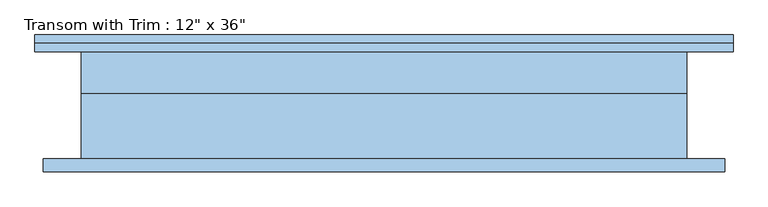
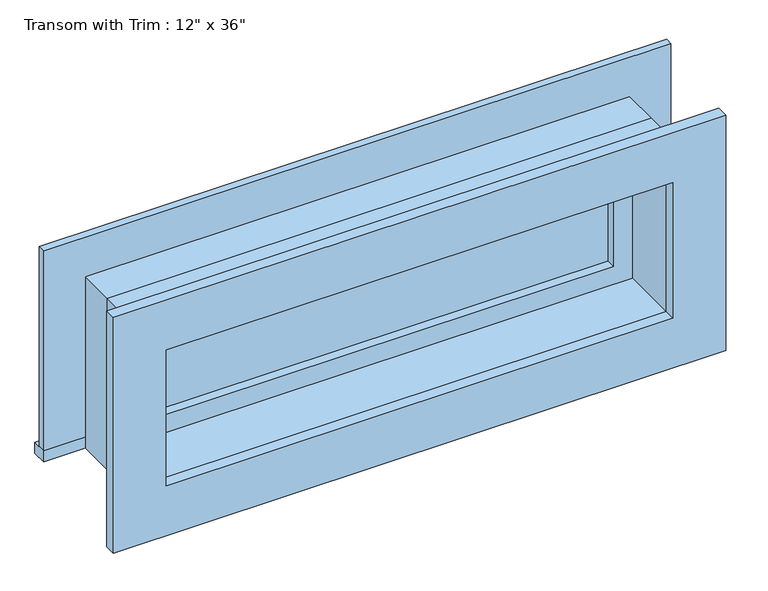
"""IFC4 building model written with IfcOpenShell, lengths in millimetres: window geometry."""

from ifc_helpers import new_model, si_unit, frame, origin, place, context, project, spatial, polyline, outline, extrude, source, transform, mapped, element, save


def window_4a3b5ce9(model_context):
    return source(origin(), model_context, "Body", "SweptSolid", [
        extrude(outline(polyline([(-565.15, 106.3625), (488.95, 106.3625), (488.95, 80.9625), (-565.15, 80.9625), (-565.15, 106.3625)])), frame((0.0, 0.0, 2159.0), z_axis=(0.0, 0.0, 1.0), x_axis=(1.0, 0.0, 0.0)), (0.0, 0.0, 1.0), 19.05),
        extrude(outline(polyline([(2444.75, -476.25), (2444.75, 400.05), (2178.05, 400.05), (2178.05, 488.95), (2533.65, 488.95), (2533.65, -565.15), (2178.05, -565.15), (2178.05, -476.25), (2444.75, -476.25)])), frame((0.0, 80.9625, 0.0), z_axis=(0.0, 1.0, 0.0), x_axis=(0.0, 0.0, 1.0)), (0.0, 0.0, 1.0), 12.7),
        extrude(outline(polyline([(2520.95, 476.25), (2520.95, -552.45), (2101.85, -552.45), (2101.85, 476.25), (2520.95, 476.25)]), holes=[polyline([(2432.05, 387.35), (2190.75, 387.35), (2190.75, -463.55), (2432.05, -463.55), (2432.05, 387.35)])]), frame((0.0, -100.0125, 0.0), z_axis=(0.0, 1.0, 0.0), x_axis=(0.0, 0.0, 1.0)), (0.0, 0.0, 1.0), 19.05),
        extrude(outline(polyline([(355.6, 33.3375), (-431.8, 33.3375), (-431.8, 46.0375), (355.6, 46.0375), (355.6, 33.3375)])), frame((0.0, 0.0, 2222.5), z_axis=(0.0, 0.0, 1.0), x_axis=(1.0, 0.0, 0.0)), (0.0, 0.0, 1.0), 177.8),
        extrude(outline(polyline([(2444.75, -476.25), (2178.05, -476.25), (2178.05, 400.05), (2444.75, 400.05), (2444.75, -476.25)]), holes=[polyline([(2400.3, -431.8), (2400.3, 355.6), (2222.5, 355.6), (2222.5, -431.8), (2400.3, -431.8)])]), frame((0.0, 17.4625, 0.0), z_axis=(0.0, 1.0, 0.0), x_axis=(0.0, 0.0, 1.0)), (0.0, 0.0, 1.0), 44.45),
        extrude(outline(polyline([(2463.8, -495.3), (2159.0, -495.3), (2159.0, 419.1), (2463.8, 419.1), (2463.8, -495.3)]), holes=[polyline([(2432.05, -463.55), (2432.05, 387.35), (2190.75, 387.35), (2190.75, -463.55), (2432.05, -463.55)])]), frame((0.0, -80.9625, 0.0), z_axis=(0.0, 1.0, 0.0), x_axis=(0.0, 0.0, 1.0)), (0.0, 0.0, 1.0), 98.425),
        extrude(outline(polyline([(2463.8, 419.1), (2463.8, -495.3), (2159.0, -495.3), (2159.0, 419.1), (2463.8, 419.1)]), holes=[polyline([(2444.75, 400.05), (2178.05, 400.05), (2178.05, -476.25), (2444.75, -476.25), (2444.75, 400.05)])]), frame((0.0, 17.4625, 0.0), z_axis=(0.0, 1.0, 0.0), x_axis=(0.0, 0.0, 1.0)), (0.0, 0.0, 1.0), 63.5),
    ])


if __name__ == "__main__":
    model = new_model("IFC4")
    model_context = context("Model", 3, world=origin())
    ifc_project = project(units=[si_unit("LENGTHUNIT", "METRE", prefix="MILLI")], contexts=[model_context])
    site = spatial("IfcSite", under=ifc_project)
    building = spatial("IfcBuilding", under=site)
    placement = place(None, origin())
    window_shape = window_4a3b5ce9(model_context)
    element("IfcWindow", 1, ObjectType="Transom with Trim : 12\" x 36\"", at=placement, inside=building, context=model_context, shape_type="MappedRepresentation", body=[
        mapped(window_shape, transform((0.0, 0.0, 0.0), x_axis=(1.0, 0.0, 0.0), y_axis=(0.0, 1.0, 0.0), z_axis=(0.0, 0.0, 1.0))),
    ])
    save(model, "model.ifc")

# Revit data of these elements
# Type "Transom with Trim : 12\" x 36\""
#   Type Mark = "40"
#   COBie.Type.CreatedBy = "doug.wood@us.ibm.com"
#   COBie.Type.CreatedOn = "2016-04-14T02:07:26"
#   COBie.Type.Name = "Windows_Transom with Trim_12\" x 36\"_40"
#   COBie.Type.Category = "23-30 20 00 : Windows"
#   COBie.Type.Description = "Transom with Trim_12\" x 36\""
#   COBie.Type.Manufacturer = ""
#   COBie.Type.ModelNumber = ""
#   Construction Type Id = "GSP4R"
#   Assembly Code = "B2020100"
#   Analytic Construction = "1/8 in Pilkington single glazing"
#   COBie.Type.ReplacementCost = 0
#   Visual Light Transmittance = 0.9
#   Solar Heat Gain Coefficient = 0.78
#   Heat Transfer Coefficient (U) = 3.6886 W/(m²·K)
#   Height = 1' - 0"
#   Default Sill Height = 7' - 1"
#   Trim Projection - Ext. = 0' - 0 1/2"
#   Trim Projection - Int. = 0' - 0 3/4"
#   Trim Width - Exterior = 0' - 3 1/2"
#   Trim Width - Interior = 0' - 3 1/2"
#   Width = 3' - 0"
#   Window Inset = 0' - 0 3/4"
#   COBie.Type = no
#   Glass Pane Material = Glass
#   Sash Material = Sash - White
#   Trim Exterior Material = Trim - White
#   Trim Interior Material = Trim - White
#   Wall Closure = (empty or 0)
# Element 1 (IfcWindow, "Transom with Trim : 12\" x 36\"")
#   Materials on its faces: "Sash - White", "Trim - White", "Glass"
# Materials
#   "Glass": class "Glass", colour RGB 0 128 192, transparency 0.75, Description = "Soda Lime Glass", Cost = 0
#   "Sash - White": class "Wood", colour RGB 255 255 255, transparency 0, Cost = 0
#   "Trim - White": class "Wood", colour RGB 255 255 255, transparency 0, Cost = 0
